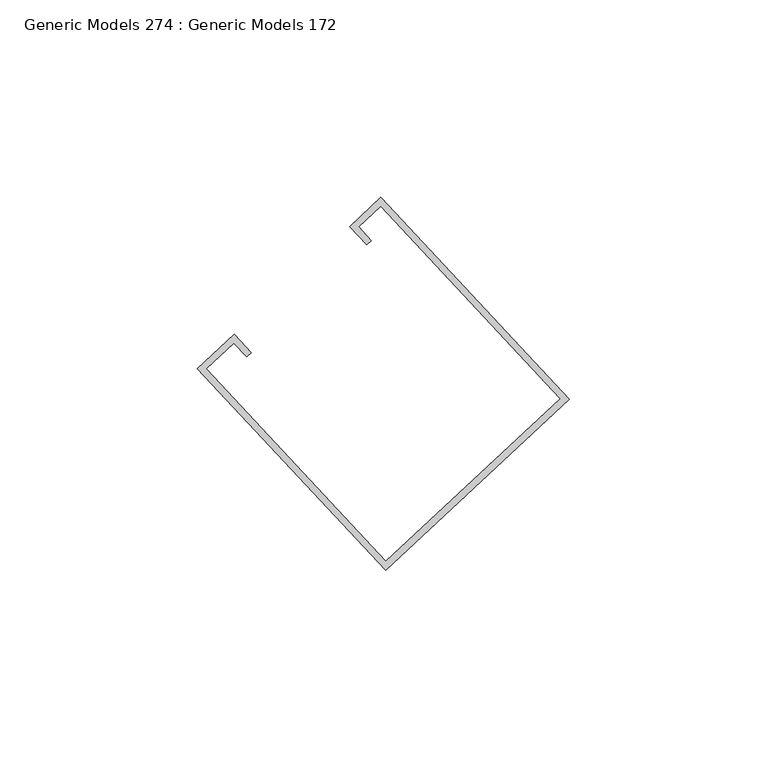
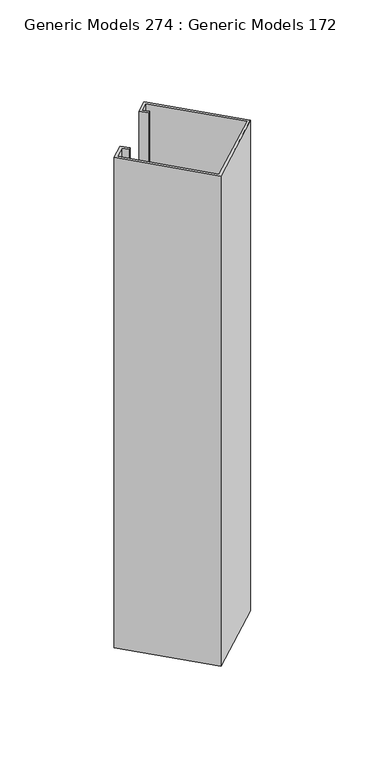
"""IFC4 building model written with IfcOpenShell, lengths in millimetres: proxy geometry, Generic Models 274 : Generic Models 172."""

from ifc_helpers import new_model, si_unit, origin, origin_with_axes, place, context, project, spatial, polyline, outline, extrude, source, transform, mapped, element, save


def generic_models_274_generic_models_172_b71e9c20(model_context):
    return source(origin(), model_context, "Body", "SweptSolid", [
        extrude(outline(polyline([(-438.6289329, -19897.2170189), (-445.5950769, -19903.7130533), (-400.1228362, -19952.4760614), (-356.0039242, -19911.3345103), (-401.4761648, -19862.5715022), (-407.0527368, -19867.7717397), (-403.8047196, -19871.2548117), (-404.9657436, -19872.3374841), (-409.2964332, -19867.6933881), (-401.3978132, -19860.3278058), (-353.7602278, -19911.4128619), (-400.2011878, -19954.7197578), (-447.8387733, -19903.6347017), (-438.5505813, -19894.9733225), (-434.2198917, -19899.6174185), (-435.3809157, -19900.7000909), (-438.6289329, -19897.2170189)])), origin_with_axes(), (0.0, 0.0, 1.0), 374.65),
    ])


if __name__ == "__main__":
    model = new_model("IFC4")
    model_context = context("Model", 3, world=origin())
    ifc_project = project(units=[si_unit("LENGTHUNIT", "METRE", prefix="MILLI")], contexts=[model_context])
    site = spatial("IfcSite", under=ifc_project)
    building = spatial("IfcBuilding", under=site)
    placement = place(None, origin())
    generic_models_274_generic_models_172_shape = generic_models_274_generic_models_172_b71e9c20(model_context)
    element("IfcBuildingElementProxy", 1, Name="Generic Models 274 : Generic Models 172", ObjectType="Generic Models 274 : Generic Models 172", at=placement, inside=building, context=model_context, shape_type="MappedRepresentation", body=[
        mapped(generic_models_274_generic_models_172_shape, transform((0.0, 0.0, 0.0), x_axis=(1.0, 0.0, 0.0), y_axis=(0.0, 1.0, 0.0), z_axis=(0.0, 0.0, 1.0))),
    ])
    save(model, "model.ifc")

# Revit data of these elements
# Element 1 (IfcBuildingElementProxy, "Generic Models 274 : Generic Models 172")
#   Materials on its faces: "GALVANIZED UNISTRUT P5500, 1 5/8\" X 2 7/16\" OR ALUM. CHANNEL"
# Materials
#   "GALVANIZED UNISTRUT P5500, 1 5/8\" X 2 7/16\" OR ALUM. CHANNEL": class "Metal", colour RGB 244 244 244, transparency 0, Description = "Aluminum 6061", Cost = 0
